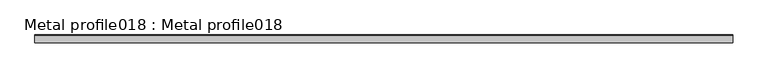
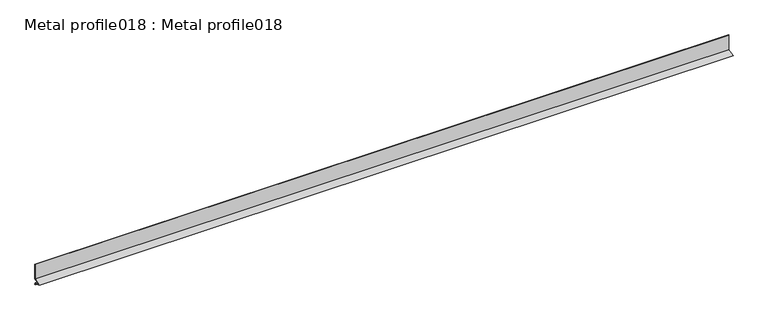
"""IFC4 building model written with IfcOpenShell, lengths in millimetres: proxy geometry, Metal profile018 : Metal profile018."""

import ifcopenshell
import ifcopenshell.guid

model = None  # the IFC model being written
_history = None  # IfcOwnerHistory: only IFC2X3 demands one
_inside = {}  # id of a spatial element -> (the spatial element, [elements in it])
_under = {}  # id of a project, library or spatial element -> (it, [spatial elements below it])
_declared = {}  # id of a project -> (the project, [libraries it declares])
_typed = {}  # id of a type object -> (the type object, [elements of that type])
_made_of = {}  # id of a material, layer set ... -> (it, [elements and type objects made of it])


def new_model(schema):
    """Start an empty IFC model of exactly this schema.

    Asked for "IFC4X3", IfcOpenShell would pick the latest addendum, in which some entities
    have other attributes; the version numbers below select the first issue.
    IFC2X3 requires an IfcOwnerHistory on every rooted entity: one is made here for all.
    """
    global model, _history
    if schema == "IFC4X3":
        model = ifcopenshell.file(schema_version=(4, 3, 0, 0))
    else:
        model = ifcopenshell.file(schema=schema)
    _inside.clear()
    _under.clear()
    _declared.clear()
    _typed.clear()
    _made_of.clear()
    _history = None
    if model.schema == "IFC2X3":
        org = make("IfcOrganization", Name="unknown")
        user = make(
            "IfcPersonAndOrganization",
            ThePerson=make("IfcPerson", FamilyName="unknown"),
            TheOrganization=org,
        )
        app = make(
            "IfcApplication",
            ApplicationDeveloper=org,
            Version="unknown",
            ApplicationFullName="unknown",
            ApplicationIdentifier="unknown",
        )
        _history = make(
            "IfcOwnerHistory",
            OwningUser=user,
            OwningApplication=app,
            ChangeAction="ADDED",
            CreationDate=0,
        )
    return model


def make(cls, **values):
    """One entity of the class cls with the attributes given. An attribute that is None is left unset."""
    return model.create_entity(
        cls, **{name: value for name, value in values.items() if value is not None}
    )


def rooted(cls, **values):
    """An entity with a GlobalId (a new one), such as an element, a storey or a relation."""
    return make(cls, GlobalId=ifcopenshell.guid.new(), OwnerHistory=_history, **values)


def si_unit(unit_type, name, prefix=None):
    """IfcSIUnit, for example si_unit("LENGTHUNIT", "METRE", prefix="MILLI")."""
    return make("IfcSIUnit", UnitType=unit_type, Prefix=prefix, Name=name)


def assignment(units):
    """IfcUnitAssignment: the units of a project."""
    return None if units is None else make("IfcUnitAssignment", Units=units)


def point(xyz):
    """IfcCartesianPoint."""
    return None if xyz is None else make("IfcCartesianPoint", Coordinates=xyz)


def direction(xyz):
    """IfcDirection."""
    return None if xyz is None else make("IfcDirection", DirectionRatios=xyz)


def frame(location, z_axis=None, x_axis=None):
    """IfcAxis2Placement3D, a coordinate frame: its origin and axes. An axis left out is left unset."""
    return make(
        "IfcAxis2Placement3D",
        Location=point(location),
        Axis=direction(z_axis),
        RefDirection=direction(x_axis),
    )


def origin():
    """The frame at (0, 0, 0) with its axes left unset."""
    return frame((0.0, 0.0, 0.0))


def place(relative_to, where):
    """IfcLocalPlacement: puts the frame where relative to a parent placement (None: the world)."""
    return make(
        "IfcLocalPlacement", PlacementRelTo=relative_to, RelativePlacement=where
    )


def context(
    kind, dimensions, precision=None, world=None, true_north=None, identifier=None
):
    """IfcGeometricRepresentationContext, for example the 3D "Model" context."""
    return make(
        "IfcGeometricRepresentationContext",
        ContextIdentifier=identifier,
        ContextType=kind,
        CoordinateSpaceDimension=dimensions,
        Precision=precision,
        WorldCoordinateSystem=world,
        TrueNorth=true_north,
    )


def project(units=None, contexts=None):
    """IfcProject with its units and contexts."""
    return rooted(
        "IfcProject",
        Name="project",
        RepresentationContexts=contexts,
        UnitsInContext=assignment(units),
    )


def spatial(cls, under=None, at=None, **own):
    """A site, building, storey or space (cls), placed at a placement, below another one or the project."""
    s = rooted(cls, ObjectPlacement=at, **own)
    if under is not None:
        _under.setdefault(under.id(), (under, []))[1].append(s)
    return s


def polyline(points):
    """IfcPolyline through the points."""
    return make("IfcPolyline", Points=[point(p) for p in points])


def outline(outer, holes=None, kind="AREA"):
    """IfcArbitraryClosedProfileDef: a profile drawn as a closed curve; with holes, ...WithVoids."""
    if holes is None:
        return make("IfcArbitraryClosedProfileDef", ProfileType=kind, OuterCurve=outer)
    return make(
        "IfcArbitraryProfileDefWithVoids",
        ProfileType=kind,
        OuterCurve=outer,
        InnerCurves=holes,
    )


def extrude(swept, where, along, depth):
    """IfcExtrudedAreaSolid: the profile swept, set in the frame where, extruded along a direction by depth."""
    return make(
        "IfcExtrudedAreaSolid",
        SweptArea=swept,
        Position=where,
        ExtrudedDirection=direction(along),
        Depth=depth,
    )


def shape(context_of_items, identifier, shape_type, items):
    """IfcShapeRepresentation: the items that make up one representation, for example the "Body"."""
    return make(
        "IfcShapeRepresentation",
        ContextOfItems=context_of_items,
        RepresentationIdentifier=identifier,
        RepresentationType=shape_type,
        Items=items,
    )


def source(mapping_origin, context_of_items, identifier, shape_type, items):
    """IfcRepresentationMap: a shape defined once, which mapped items show again and again."""
    return make(
        "IfcRepresentationMap",
        MappingOrigin=mapping_origin,
        MappedRepresentation=shape(context_of_items, identifier, shape_type, items),
    )


def transform(
    local_origin,
    x_axis=None,
    y_axis=None,
    z_axis=None,
    scale=None,
    scale2=None,
    scale3=None,
    uniform=True,
):
    """IfcCartesianTransformationOperator3D, or its non-uniform kind. x_axis, y_axis, z_axis: its Axis1, 2, 3."""
    if uniform:
        return make(
            "IfcCartesianTransformationOperator3D",
            Axis1=direction(x_axis),
            Axis2=direction(y_axis),
            LocalOrigin=point(local_origin),
            Scale=scale,
            Axis3=direction(z_axis),
        )
    return make(
        "IfcCartesianTransformationOperator3DnonUniform",
        Axis1=direction(x_axis),
        Axis2=direction(y_axis),
        LocalOrigin=point(local_origin),
        Scale=scale,
        Axis3=direction(z_axis),
        Scale2=scale2,
        Scale3=scale3,
    )


def mapped(mapping_source, mapping_target):
    """IfcMappedItem: shows the shape of a source again, moved by a transform."""
    return make(
        "IfcMappedItem", MappingSource=mapping_source, MappingTarget=mapping_target
    )


def made_of(thing, what):
    """Note that an element or type object is made of a material, layer set ...; save() writes the relation."""
    if what is not None:
        _made_of.setdefault(what.id(), (what, []))[1].append(thing)
    return thing


def element(
    cls,
    number,
    at=None,
    inside=None,
    cuts=None,
    type_object=None,
    material=None,
    context=None,
    identifier="Body",
    shape_type=None,
    held_by="IfcProductDefinitionShape",
    body=None,
    shapes=None,
    **own,
):
    """One element of the class cls, such as IfcWall. Its Tag is "e" and its number.

    at: its placement. inside: the storey or other place that contains it. cuts: it is an
    opening in that element (IfcRelVoidsElement). A single representation is given by context,
    identifier, shape_type and body (its items); several are given by shapes. held_by: the class
    of the entity that holds the representations. save() writes the other relations.
    """
    e = rooted(cls, Tag="e%d" % number, ObjectPlacement=at, **own)
    if body is not None:
        shapes = [shape(context, identifier, shape_type, body)]
    if shapes is not None:
        e.Representation = make(held_by, Representations=shapes)
    if inside is not None:
        _inside.setdefault(inside.id(), (inside, []))[1].append(e)
    if cuts is not None:
        rooted(
            "IfcRelVoidsElement", RelatingBuildingElement=cuts, RelatedOpeningElement=e
        )
    if type_object is not None:
        _typed.setdefault(type_object.id(), (type_object, []))[1].append(e)
    return made_of(e, material)


def aggregate(whole, parts):
    """IfcRelAggregates: a whole, such as a stair, and the parts it consists of."""
    return rooted("IfcRelAggregates", RelatingObject=whole, RelatedObjects=parts)


def save(model, path):
    """Write the relations noted so far, then the file.

    IfcRelAggregates (storeys below a building ...), IfcRelContainedInSpatialStructure (elements
    in a storey), IfcRelDefinesByType, IfcRelAssociatesMaterial and IfcRelDeclares: one each for
    every whole, place, type object, material and project.
    """
    for whole, parts in _under.values():
        aggregate(whole, parts)
    for where, things in _inside.values():
        rooted(
            "IfcRelContainedInSpatialStructure",
            RelatedElements=things,
            RelatingStructure=where,
        )
    for kind, things in _typed.values():
        rooted("IfcRelDefinesByType", RelatedObjects=things, RelatingType=kind)
    for what, things in _made_of.values():
        rooted("IfcRelAssociatesMaterial", RelatedObjects=things, RelatingMaterial=what)
    for by, libraries in _declared.values():
        rooted("IfcRelDeclares", RelatingContext=by, RelatedDefinitions=libraries)
    model.write(path)


def metal_profile018_metal_profile018_7e7df4c7(model_context):
    return source(origin(), model_context, "Body", "SweptSolid", [
        extrude(outline(polyline([(-4659.7667972, 36534.5192167), (-4661.0148598, 36534.2841851), (-4661.8381807, 36538.6561768), (-4681.9917972, 36545.134125), (-4661.0367972, 36551.8696607), (-4661.0367972, 36595.934125), (-4659.7667972, 36595.934125), (-4659.7667972, 36550.9438814), (-4677.8415949, 36545.134125), (-4660.7299923, 36539.633967), (-4659.7667972, 36534.5192167)])), frame((12383.0178845, 0.0, 0.0), z_axis=(1.0, 0.0, 0.0), x_axis=(0.0, 1.0, 0.0)), (0.0, 0.0, 1.0), 2000.0),
    ])


if __name__ == "__main__":
    model = new_model("IFC4")
    model_context = context("Model", 3, world=origin())
    ifc_project = project(units=[si_unit("LENGTHUNIT", "METRE", prefix="MILLI")], contexts=[model_context])
    site = spatial("IfcSite", under=ifc_project)
    building = spatial("IfcBuilding", under=site)
    placement = place(None, origin())
    metal_profile018_metal_profile018_shape = metal_profile018_metal_profile018_7e7df4c7(model_context)
    element("IfcBuildingElementProxy", 1, Name="Metal profile018 : Metal profile018", ObjectType="Metal profile018 : Metal profile018", at=placement, inside=building, context=model_context, shape_type="MappedRepresentation", body=[
        mapped(metal_profile018_metal_profile018_shape, transform((0.0, 0.0, 0.0), x_axis=(1.0, 0.0, 0.0), y_axis=(0.0, 1.0, 0.0), z_axis=(0.0, 0.0, 1.0))),
    ])
    save(model, "model.ifc")

# Revit data of these elements
# Type "Metal profile018 : Metal profile018"
#   NameOverride = "Metal profile018"
# Element 1 (IfcBuildingElementProxy, "Metal profile018 : Metal profile018")
#   Materials on its faces: "16 GA. COPPER WEEP SCREED W/ MIN 3 1/2\" ATTACHMENT FLANGE - LAP UNDERLAYMENT OVER WEED SCREED"
# Materials
#   "16 GA. COPPER WEEP SCREED W/ MIN 3 1/2\" ATTACHMENT FLANGE - LAP UNDERLAYMENT OVER WEED SCREED": class "Unassigned", colour RGB 251 232 155, transparency 0, Cost = 0
